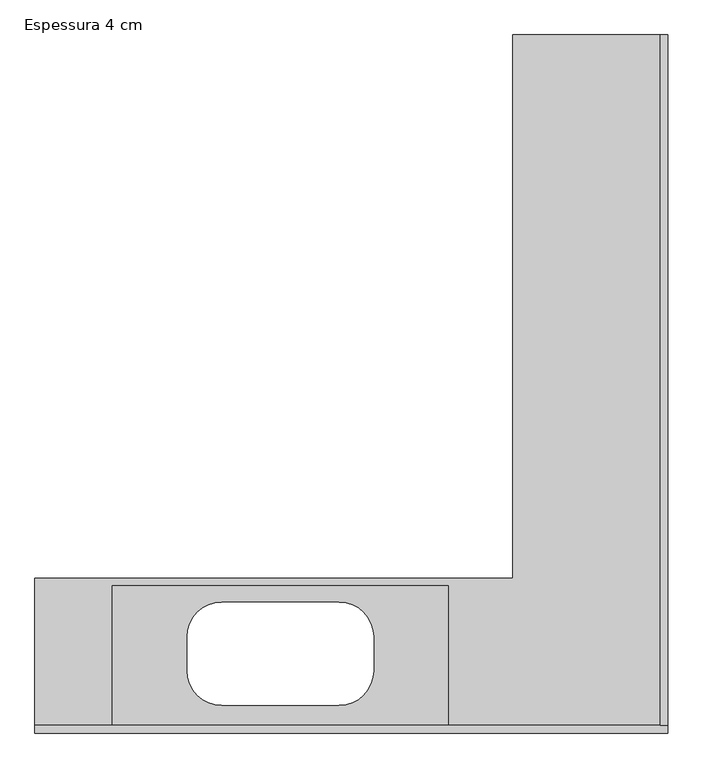
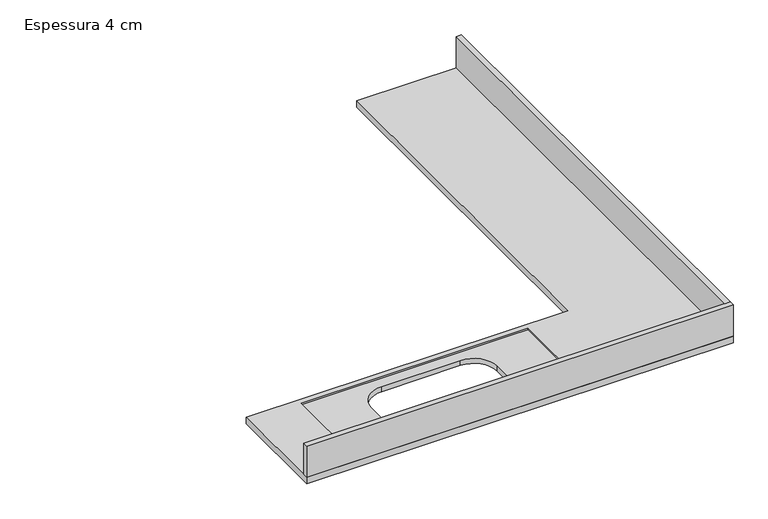
"""IFC4 building model written with IfcOpenShell, lengths in millimetres: furniture geometry, .BANCADA EM L_COZINHA_CUBA DUPLA : Espessura 4 cm."""

from ifc_helpers import new_model, si_unit, frame, origin, place, context, project, spatial, polyline, circle_curve, outline, extrude, source, transform, mapped, element, save
from ifc_brep_helpers import plane_surface, revolved_surface, advanced_brep


def espessura_4_cm_91f9314f(model_context):
    return source(origin(), model_context, "Body", "SolidModel", [
        extrude(outline(polyline([(-30.0, 30.0), (-30.0, 2702.2838598), (0.0, 2702.2838598), (0.0, 30.0), (-30.0, 30.0)])), frame((0.0, 0.0, 900.0), z_axis=(0.0, 0.0, 1.0), x_axis=(1.0, 0.0, 0.0)), (0.0, 0.0, 1.0), 190.0),
        extrude(outline(polyline([(-2449.7786374, 30.0), (0.0, 30.0), (0.0, 0.0), (-2449.7786374, 0.0), (-2449.7786374, 30.0)])), frame((0.0, 0.0, 900.0), z_axis=(0.0, 0.0, 1.0), x_axis=(1.0, 0.0, 0.0)), (0.0, 0.0, 1.0), 190.0),
        advanced_brep(
        [(-600.0, 600.0, 860.0), (-600.0, 2702.2838598, 860.0), (0.0, 2702.2838598, 860.0), (0.0, 0.0, 860.0), (-2449.7786374, 0.0, 860.0), (-2449.7786374, 600.0, 860.0), (-1725.7786374, 107.0, 860.0), (-1273.7786374, 107.0, 860.0), (-1138.7786374, 242.0, 860.0), (-1138.7786374, 372.0, 860.0), (-1273.7786374, 507.0, 860.0), (-1725.7786374, 507.0, 860.0), (-1860.7786374, 372.0, 860.0), (-1860.7786374, 242.0, 860.0), (-600.0, 600.0, 900.0), (-2449.7786374, 600.0, 900.0), (-2449.7786374, 0.0, 900.0), (0.0, 0.0, 900.0), (0.0, 2702.2838598, 900.0), (-600.0, 2702.2838598, 900.0), (-849.7786374, 30.0, 900.0), (-2149.7786374, 30.0, 900.0), (-2149.7786374, 570.0, 900.0), (-849.7786374, 570.0, 900.0), (-1725.7786374, 107.0, 890.0), (-1273.7786374, 107.0, 890.0), (-1138.7786374, 242.0, 890.0), (-1138.7786374, 372.0, 890.0), (-1273.7786374, 507.0, 890.0), (-1725.7786374, 507.0, 890.0), (-1860.7786374, 372.0, 890.0), (-1860.7786374, 242.0, 890.0), (-849.7786374, 570.0, 890.0), (-2149.7786374, 570.0, 890.0), (-2149.7786374, 30.0, 890.0), (-849.7786374, 30.0, 890.0)],
        [
            (0, 1),
            (1, 2),
            (2, 3),
            (3, 4),
            (4, 5),
            (5, 0),
            (6, 7),
            (7, 8, circle_curve(frame((-1273.7786374, 242.0, 860.0), z_axis=(0.0, 0.0, 1.0), x_axis=(-1.0, 0.0, 0.0)), 135.0)),
            (8, 9),
            (9, 10, circle_curve(frame((-1273.7786374, 372.0, 860.0), z_axis=(0.0, 0.0, 1.0), x_axis=(-1.0, 0.0, 0.0)), 135.0)),
            (10, 11),
            (11, 12, circle_curve(frame((-1725.7786374, 372.0, 860.0), z_axis=(0.0, 0.0, 1.0), x_axis=(-1.0, 0.0, 0.0)), 135.0)),
            (12, 13),
            (13, 6, circle_curve(frame((-1725.7786374, 242.0, 860.0), z_axis=(0.0, 0.0, 1.0), x_axis=(-1.0, 0.0, 0.0)), 135.0)),
            (14, 15),
            (15, 16),
            (16, 17),
            (17, 18),
            (18, 19),
            (19, 14),
            (20, 21),
            (21, 22),
            (22, 23),
            (23, 20),
            (0, 14),
            (19, 1),
            (18, 2),
            (17, 3),
            (16, 4),
            (15, 5),
            (6, 24),
            (24, 25),
            (25, 7),
            (25, 26, circle_curve(frame((-1273.7786374, 242.0, 890.0), z_axis=(0.0, 0.0, 1.0), x_axis=(-1.0, 0.0, 0.0)), 135.0)),
            (26, 8),
            (26, 27),
            (27, 9),
            (27, 28, circle_curve(frame((-1273.7786374, 372.0, 890.0), z_axis=(0.0, 0.0, 1.0), x_axis=(-1.0, 0.0, 0.0)), 135.0)),
            (28, 10),
            (28, 29),
            (29, 11),
            (29, 30, circle_curve(frame((-1725.7786374, 372.0, 890.0), z_axis=(0.0, 0.0, 1.0), x_axis=(-1.0, 0.0, 0.0)), 135.0)),
            (30, 12),
            (30, 31),
            (31, 13),
            (31, 24, circle_curve(frame((-1725.7786374, 242.0, 890.0), z_axis=(0.0, 0.0, 1.0), x_axis=(-1.0, 0.0, 0.0)), 135.0)),
            (32, 33),
            (33, 34),
            (34, 35),
            (35, 32),
            (35, 20),
            (23, 32),
            (34, 21),
            (33, 22),
        ],
        [
            plane_surface(frame((-600.0, 600.0, 860.0), z_axis=(0.0, 0.0, -1.0), x_axis=(0.0, -1.0, 0.0))),
            plane_surface(frame((-600.0, 600.0, 900.0), z_axis=(0.0, 0.0, 1.0), x_axis=(0.0, 1.0, 0.0))),
            plane_surface(frame((-600.0, 600.0, 900.0), z_axis=(-1.0, 0.0, 0.0), x_axis=(0.0, 0.0, -1.0))),
            plane_surface(frame((-600.0, 2702.2838598, 900.0), z_axis=(0.0, 1.0, 0.0), x_axis=(0.0, 0.0, -1.0))),
            plane_surface(frame((0.0, 2702.2838598, 900.0), z_axis=(1.0, 0.0, 0.0), x_axis=(0.0, 0.0, -1.0))),
            plane_surface(frame((0.0, 0.0, 900.0), z_axis=(0.0, -1.0, 0.0), x_axis=(0.0, 0.0, -1.0))),
            plane_surface(frame((-2449.7786374, 0.0, 900.0), z_axis=(-1.0, 0.0, 0.0), x_axis=(0.0, 0.0, -1.0))),
            plane_surface(frame((-2449.7786374, 600.0, 900.0), z_axis=(0.0, 1.0, 0.0), x_axis=(0.0, 0.0, -1.0))),
            plane_surface(frame((-1725.7786374, 107.0, 900.0), z_axis=(0.0, 1.0, 0.0), x_axis=(0.0, 0.0, -1.0))),
            revolved_surface(polyline([(-1408.7786374, 242.0, 860.0), (-1408.7786374, 242.0, 890.0)]), (-1273.7786374, 242.0, 890.0), (0.0, 0.0, -1.0)),
            plane_surface(frame((-1138.7786374, 242.0, 900.0), z_axis=(-1.0, 0.0, 0.0), x_axis=(0.0, 0.0, -1.0))),
            revolved_surface(polyline([(-1408.7786374, 372.0, 860.0), (-1408.7786374, 372.0, 890.0)]), (-1273.7786374, 372.0, 890.0), (0.0, 0.0, -1.0)),
            plane_surface(frame((-1273.7786374, 507.0, 900.0), z_axis=(0.0, -1.0, 0.0), x_axis=(0.0, 0.0, -1.0))),
            revolved_surface(polyline([(-1860.7786374, 372.0, 860.0), (-1860.7786374, 372.0, 890.0)]), (-1725.7786374, 372.0, 890.0), (0.0, 0.0, -1.0)),
            plane_surface(frame((-1860.7786374, 372.0, 900.0), z_axis=(1.0, 0.0, 0.0), x_axis=(0.0, 0.0, -1.0))),
            revolved_surface(polyline([(-1860.7786374, 242.0, 860.0), (-1860.7786374, 242.0, 890.0)]), (-1725.7786374, 242.0, 890.0), (0.0, 0.0, -1.0)),
            plane_surface(frame((-849.7786374, 30.0, 890.0), z_axis=(0.0, 0.0, 1.0), x_axis=(0.0, 1.0, 0.0))),
            plane_surface(frame((-849.7786374, 570.0, 940.0), z_axis=(-1.0, 0.0, 0.0), x_axis=(0.0, 0.0, -1.0))),
            plane_surface(frame((-849.7786374, 30.0, 940.0), z_axis=(0.0, 1.0, 0.0), x_axis=(0.0, 0.0, -1.0))),
            plane_surface(frame((-2149.7786374, 30.0, 940.0), z_axis=(1.0, 0.0, 0.0), x_axis=(0.0, 0.0, -1.0))),
            plane_surface(frame((-2149.7786374, 570.0, 940.0), z_axis=(0.0, -1.0, 0.0), x_axis=(0.0, 0.0, -1.0))),
        ],
        [
            (0, [[1, 2, 3, 4, 5, 6], [7, 8, 9, 10, 11, 12, 13, 14]]),
            (1, [[15, 16, 17, 18, 19, 20], [21, 22, 23, 24]]),
            (2, [[25, -20, 26, -1]]),
            (3, [[-26, -19, 27, -2]]),
            (4, [[-27, -18, 28, -3]]),
            (5, [[-28, -17, 29, -4]]),
            (6, [[-29, -16, 30, -5]]),
            (7, [[-30, -15, -25, -6]]),
            (8, [[31, 32, 33, -7]]),
            (9, [[-33, 34, 35, -8]]),
            (10, [[-35, 36, 37, -9]]),
            (11, [[-37, 38, 39, -10]]),
            (12, [[-39, 40, 41, -11]]),
            (13, [[-41, 42, 43, -12]]),
            (14, [[-43, 44, 45, -13]]),
            (15, [[-45, 46, -31, -14]]),
            (16, [[47, 48, 49, 50], [-46, -44, -42, -40, -38, -36, -34, -32]]),
            (17, [[51, -24, 52, -50]]),
            (18, [[53, -21, -51, -49]]),
            (19, [[54, -22, -53, -48]]),
            (20, [[-52, -23, -54, -47]]),
        ],
    ),
    ])


if __name__ == "__main__":
    model = new_model("IFC4")
    model_context = context("Model", 3, world=origin())
    ifc_project = project(units=[si_unit("LENGTHUNIT", "METRE", prefix="MILLI")], contexts=[model_context])
    site = spatial("IfcSite", under=ifc_project)
    building = spatial("IfcBuilding", under=site)
    placement = place(None, origin())
    espessura_4_cm_shape = espessura_4_cm_91f9314f(model_context)
    element("IfcFurniture", 1, ObjectType=".BANCADA EM L_COZINHA_CUBA DUPLA : Espessura 4 cm", at=placement, inside=building, context=model_context, shape_type="MappedRepresentation", body=[
        mapped(espessura_4_cm_shape, transform((0.0, 0.0, 0.0), x_axis=(1.0, 0.0, 0.0), y_axis=(0.0, 1.0, 0.0), z_axis=(0.0, 0.0, 1.0))),
    ])
    save(model, "model.ifc")

# Revit data of these elements
# Type ".BANCADA EM L_COZINHA_CUBA DUPLA : Espessura 4 cm"
#   Offset esq área molhada [instance default] = 0.80 m
#   Largura área molhada [instance default] = 1.50 m
#   Largura principal [instance default] = 0.60 m
#   Largura da extensão [instance default] = 0.50 m
#   Espessura total da bancada [instance default] = 0.04 m
#   Espessura do frontão [instance default] = 0.03 m
#   Dist. cuba - borda [instance default] = 0.07 m
#   Compr. total principal [instance default] = 3.95 m
#   Compr. principal [instance default] = 3.45 m
#   Compr. total extensão [instance default] = 1.50 m
#   Compr. extensão [instance default] = 0.90 m
#   Altura do rebaixo da área molhada [instance default] = 0.01 m
#   Altura do frontão [instance default] = 0.20 m
#   Altura da bancada [instance default] = 0.90 m
#   Frontão fundos principal [instance default] = yes
#   Frontão fundos extensão [instance default] = yes
#   Frontão esquerdo principal [instance default] = yes
#   Frontão direito extensão [instance default] = yes
#   Material da bancada [instance default] = none
# Element 1 (IfcFurniture, ".BANCADA EM L_COZINHA_CUBA DUPLA : Espessura 4 cm")
#   Offset esq área molhada = 0.30 m
#   Largura área molhada = 1.30 m
#   Largura da extensão = 0.60 m
#   Compr. total principal = 2.449779 m
#   Compr. principal = 1.849779 m
#   Compr. total extensão = 2.702284 m
#   Compr. extensão = 2.102284 m
#   Frontão esquerdo principal = no
#   Frontão direito extensão = no
#   Material da bancada = .GRANITO BRANCO ITAUNAS
#   Materials on its faces: ".GRANITO BRANCO ITAUNAS"
# Materials
#   ".GRANITO BRANCO ITAUNAS": class ".CC_PEDRA REVEST.", colour RGB 202 195 174, transparency 0, Description = "Revestimento em granito", Cost = 0
